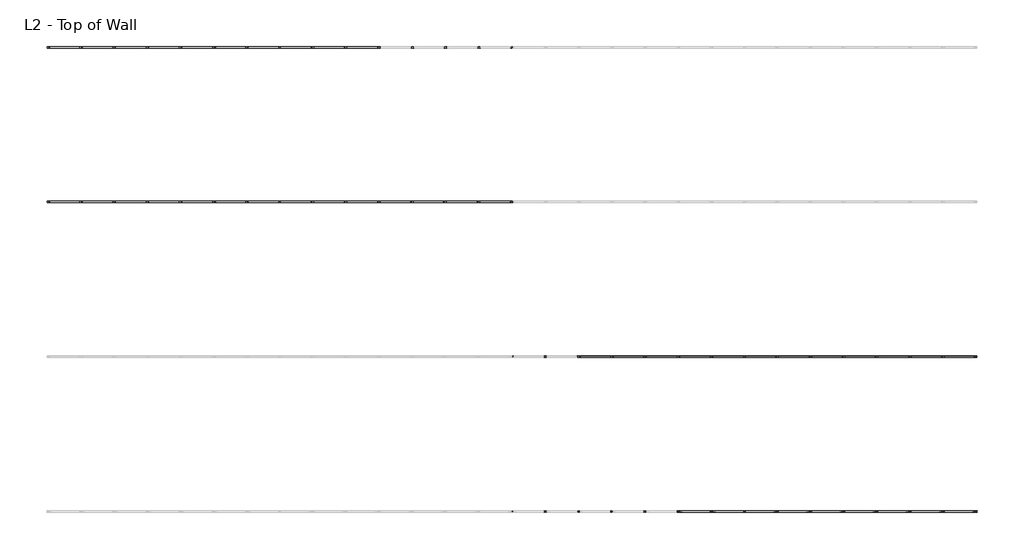
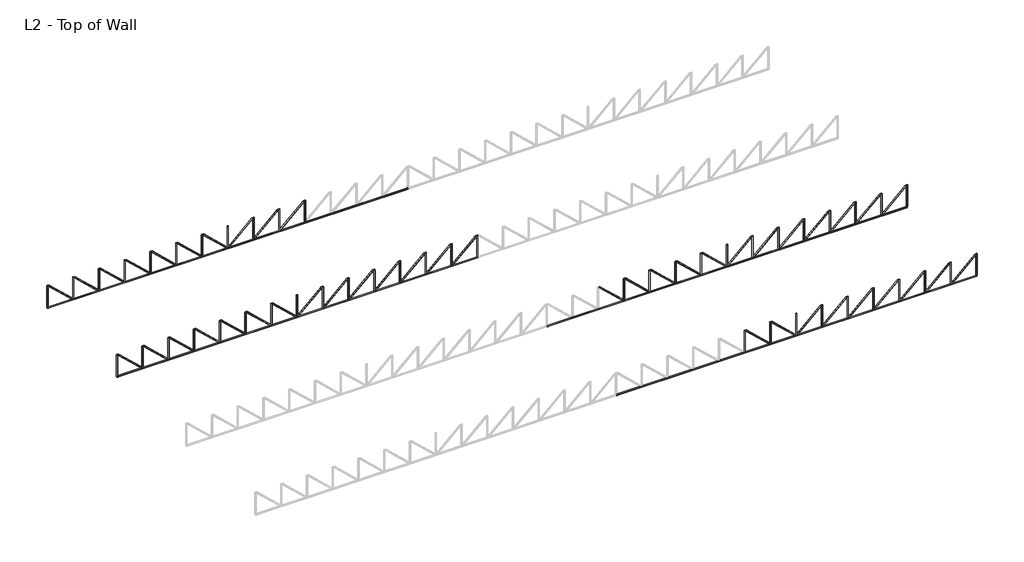
# One storey, part 3 of 4: 97 beams.
"""IFC4 building model written with IfcOpenShell, lengths in millimetres."""

import ifcopenshell
import ifcopenshell.guid

model = None  # the IFC model being written
_history = None  # IfcOwnerHistory: only IFC2X3 demands one
_inside = {}  # id of a spatial element -> (the spatial element, [elements in it])
_under = {}  # id of a project, library or spatial element -> (it, [spatial elements below it])
_declared = {}  # id of a project -> (the project, [libraries it declares])
_typed = {}  # id of a type object -> (the type object, [elements of that type])
_made_of = {}  # id of a material, layer set ... -> (it, [elements and type objects made of it])


def new_model(schema):
    """Start an empty IFC model of exactly this schema.

    Asked for "IFC4X3", IfcOpenShell would pick the latest addendum, in which some entities
    have other attributes; the version numbers below select the first issue.
    IFC2X3 requires an IfcOwnerHistory on every rooted entity: one is made here for all.
    """
    global model, _history
    if schema == "IFC4X3":
        model = ifcopenshell.file(schema_version=(4, 3, 0, 0))
    else:
        model = ifcopenshell.file(schema=schema)
    _inside.clear()
    _under.clear()
    _declared.clear()
    _typed.clear()
    _made_of.clear()
    _history = None
    if model.schema == "IFC2X3":
        org = make("IfcOrganization", Name="unknown")
        user = make(
            "IfcPersonAndOrganization",
            ThePerson=make("IfcPerson", FamilyName="unknown"),
            TheOrganization=org,
        )
        app = make(
            "IfcApplication",
            ApplicationDeveloper=org,
            Version="unknown",
            ApplicationFullName="unknown",
            ApplicationIdentifier="unknown",
        )
        _history = make(
            "IfcOwnerHistory",
            OwningUser=user,
            OwningApplication=app,
            ChangeAction="ADDED",
            CreationDate=0,
        )
    return model


def make(cls, **values):
    """One entity of the class cls with the attributes given. An attribute that is None is left unset."""
    return model.create_entity(
        cls, **{name: value for name, value in values.items() if value is not None}
    )


def rooted(cls, **values):
    """An entity with a GlobalId (a new one), such as an element, a storey or a relation."""
    return make(cls, GlobalId=ifcopenshell.guid.new(), OwnerHistory=_history, **values)


def si_unit(unit_type, name, prefix=None):
    """IfcSIUnit, for example si_unit("LENGTHUNIT", "METRE", prefix="MILLI")."""
    return make("IfcSIUnit", UnitType=unit_type, Prefix=prefix, Name=name)


def assignment(units):
    """IfcUnitAssignment: the units of a project."""
    return None if units is None else make("IfcUnitAssignment", Units=units)


def point(xyz):
    """IfcCartesianPoint."""
    return None if xyz is None else make("IfcCartesianPoint", Coordinates=xyz)


def direction(xyz):
    """IfcDirection."""
    return None if xyz is None else make("IfcDirection", DirectionRatios=xyz)


def frame(location, z_axis=None, x_axis=None):
    """IfcAxis2Placement3D, a coordinate frame: its origin and axes. An axis left out is left unset."""
    return make(
        "IfcAxis2Placement3D",
        Location=point(location),
        Axis=direction(z_axis),
        RefDirection=direction(x_axis),
    )


def frame_2d(location, x_axis=None):
    """IfcAxis2Placement2D, a coordinate frame in the plane: its origin and x axis."""
    return make(
        "IfcAxis2Placement2D", Location=point(location), RefDirection=direction(x_axis)
    )


def origin():
    """The frame at (0, 0, 0) with its axes left unset."""
    return frame((0.0, 0.0, 0.0))


def origin_2d():
    """The frame at (0, 0) in the plane with its x axis left unset."""
    return frame_2d((0.0, 0.0))


def place(relative_to, where):
    """IfcLocalPlacement: puts the frame where relative to a parent placement (None: the world)."""
    return make(
        "IfcLocalPlacement", PlacementRelTo=relative_to, RelativePlacement=where
    )


def context(
    kind, dimensions, precision=None, world=None, true_north=None, identifier=None
):
    """IfcGeometricRepresentationContext, for example the 3D "Model" context."""
    return make(
        "IfcGeometricRepresentationContext",
        ContextIdentifier=identifier,
        ContextType=kind,
        CoordinateSpaceDimension=dimensions,
        Precision=precision,
        WorldCoordinateSystem=world,
        TrueNorth=true_north,
    )


def project(units=None, contexts=None):
    """IfcProject with its units and contexts."""
    return rooted(
        "IfcProject",
        Name="project",
        RepresentationContexts=contexts,
        UnitsInContext=assignment(units),
    )


def spatial(cls, under=None, at=None, **own):
    """A site, building, storey or space (cls), placed at a placement, below another one or the project."""
    s = rooted(cls, ObjectPlacement=at, **own)
    if under is not None:
        _under.setdefault(under.id(), (under, []))[1].append(s)
    return s


def circle_curve(where, radius):
    """IfcCircle in the frame where."""
    return make("IfcCircle", Position=where, Radius=radius)


def trimmed(basis, trim1, trim2, sense, master):
    """IfcTrimmedCurve: the piece of a basis curve between two trims."""
    return make(
        "IfcTrimmedCurve",
        BasisCurve=basis,
        Trim1=trim1,
        Trim2=trim2,
        SenseAgreement=sense,
        MasterRepresentation=master,
    )


def segment(curve, same_sense, transition):
    """IfcCompositeCurveSegment."""
    return make(
        "IfcCompositeCurveSegment",
        Transition=transition,
        SameSense=same_sense,
        ParentCurve=curve,
    )


def composite_curve(segments, self_intersect=None):
    """IfcCompositeCurve: segments joined end to end."""
    return make("IfcCompositeCurve", Segments=segments, SelfIntersect=self_intersect)


def outline(outer, holes=None, kind="AREA"):
    """IfcArbitraryClosedProfileDef: a profile drawn as a closed curve; with holes, ...WithVoids."""
    if holes is None:
        return make("IfcArbitraryClosedProfileDef", ProfileType=kind, OuterCurve=outer)
    return make(
        "IfcArbitraryProfileDefWithVoids",
        ProfileType=kind,
        OuterCurve=outer,
        InnerCurves=holes,
    )


def extrude(swept, where, along, depth):
    """IfcExtrudedAreaSolid: the profile swept, set in the frame where, extruded along a direction by depth."""
    return make(
        "IfcExtrudedAreaSolid",
        SweptArea=swept,
        Position=where,
        ExtrudedDirection=direction(along),
        Depth=depth,
    )


def shape(context_of_items, identifier, shape_type, items):
    """IfcShapeRepresentation: the items that make up one representation, for example the "Body"."""
    return make(
        "IfcShapeRepresentation",
        ContextOfItems=context_of_items,
        RepresentationIdentifier=identifier,
        RepresentationType=shape_type,
        Items=items,
    )


def source(mapping_origin, context_of_items, identifier, shape_type, items):
    """IfcRepresentationMap: a shape defined once, which mapped items show again and again."""
    return make(
        "IfcRepresentationMap",
        MappingOrigin=mapping_origin,
        MappedRepresentation=shape(context_of_items, identifier, shape_type, items),
    )


def transform(
    local_origin,
    x_axis=None,
    y_axis=None,
    z_axis=None,
    scale=None,
    scale2=None,
    scale3=None,
    uniform=True,
):
    """IfcCartesianTransformationOperator3D, or its non-uniform kind. x_axis, y_axis, z_axis: its Axis1, 2, 3."""
    if uniform:
        return make(
            "IfcCartesianTransformationOperator3D",
            Axis1=direction(x_axis),
            Axis2=direction(y_axis),
            LocalOrigin=point(local_origin),
            Scale=scale,
            Axis3=direction(z_axis),
        )
    return make(
        "IfcCartesianTransformationOperator3DnonUniform",
        Axis1=direction(x_axis),
        Axis2=direction(y_axis),
        LocalOrigin=point(local_origin),
        Scale=scale,
        Axis3=direction(z_axis),
        Scale2=scale2,
        Scale3=scale3,
    )


def mapped(mapping_source, mapping_target):
    """IfcMappedItem: shows the shape of a source again, moved by a transform."""
    return make(
        "IfcMappedItem", MappingSource=mapping_source, MappingTarget=mapping_target
    )


def made_of(thing, what):
    """Note that an element or type object is made of a material, layer set ...; save() writes the relation."""
    if what is not None:
        _made_of.setdefault(what.id(), (what, []))[1].append(thing)
    return thing


def element(
    cls,
    number,
    at=None,
    inside=None,
    cuts=None,
    type_object=None,
    material=None,
    context=None,
    identifier="Body",
    shape_type=None,
    held_by="IfcProductDefinitionShape",
    body=None,
    shapes=None,
    **own,
):
    """One element of the class cls, such as IfcWall. Its Tag is "e" and its number.

    at: its placement. inside: the storey or other place that contains it. cuts: it is an
    opening in that element (IfcRelVoidsElement). A single representation is given by context,
    identifier, shape_type and body (its items); several are given by shapes. held_by: the class
    of the entity that holds the representations. save() writes the other relations.
    """
    e = rooted(cls, Tag="e%d" % number, ObjectPlacement=at, **own)
    if body is not None:
        shapes = [shape(context, identifier, shape_type, body)]
    if shapes is not None:
        e.Representation = make(held_by, Representations=shapes)
    if inside is not None:
        _inside.setdefault(inside.id(), (inside, []))[1].append(e)
    if cuts is not None:
        rooted(
            "IfcRelVoidsElement", RelatingBuildingElement=cuts, RelatedOpeningElement=e
        )
    if type_object is not None:
        _typed.setdefault(type_object.id(), (type_object, []))[1].append(e)
    return made_of(e, material)


def aggregate(whole, parts):
    """IfcRelAggregates: a whole, such as a stair, and the parts it consists of."""
    return rooted("IfcRelAggregates", RelatingObject=whole, RelatedObjects=parts)


def save(model, path):
    """Write the relations noted so far, then the file.

    IfcRelAggregates (storeys below a building ...), IfcRelContainedInSpatialStructure (elements
    in a storey), IfcRelDefinesByType, IfcRelAssociatesMaterial and IfcRelDeclares: one each for
    every whole, place, type object, material and project.
    """
    for whole, parts in _under.values():
        aggregate(whole, parts)
    for where, things in _inside.values():
        rooted(
            "IfcRelContainedInSpatialStructure",
            RelatedElements=things,
            RelatingStructure=where,
        )
    for kind, things in _typed.values():
        rooted("IfcRelDefinesByType", RelatedObjects=things, RelatingType=kind)
    for what, things in _made_of.values():
        rooted("IfcRelAssociatesMaterial", RelatedObjects=things, RelatingMaterial=what)
    for by, libraries in _declared.values():
        rooted("IfcRelDeclares", RelatingContext=by, RelatedDefinitions=libraries)
    model.write(path)


def circular_hollow_sections_chs60_3x5_c94bd862(model_context):
    return source(origin(), model_context, "Body", "SweptSolid", [
        extrude(outline(composite_curve([segment(trimmed(circle_curve(origin_2d(), 30.15), [point((-30.15, 0.0))], [point((30.15, 0.0))], False, "CARTESIAN"), True, "CONTINUOUS"), segment(trimmed(circle_curve(origin_2d(), 30.15), [point((30.15, 0.0))], [point((-30.15, 0.0))], False, "CARTESIAN"), True, "CONTINUOUS")], self_intersect=False), holes=[composite_curve([segment(trimmed(circle_curve(origin_2d(), 25.15), [point((25.15, 0.0))], [point((-25.15, 0.0))], True, "CARTESIAN"), True, "CONTINUOUS"), segment(trimmed(circle_curve(origin_2d(), 25.15), [point((-25.15, 0.0))], [point((25.15, 0.0))], True, "CARTESIAN"), True, "CONTINUOUS")], self_intersect=False)]), frame((-557.0, 0.0, 0.0), z_axis=(1.0, 0.0, 0.0), x_axis=(0.0, 1.0, 0.0)), (0.0, 0.0, 1.0), 1114.0),
    ])


def circular_hollow_sections_chs60_3x5_b8a643cb(model_context):
    return source(origin(), model_context, "Body", "SweptSolid", [
        extrude(outline(composite_curve([segment(trimmed(circle_curve(origin_2d(), 30.15), [point((-30.15, 0.0))], [point((30.15, 0.0))], False, "CARTESIAN"), True, "CONTINUOUS"), segment(trimmed(circle_curve(origin_2d(), 30.15), [point((30.15, 0.0))], [point((-30.15, 0.0))], False, "CARTESIAN"), True, "CONTINUOUS")], self_intersect=False), holes=[composite_curve([segment(trimmed(circle_curve(origin_2d(), 25.15), [point((25.15, 0.0))], [point((-25.15, 0.0))], True, "CARTESIAN"), True, "CONTINUOUS"), segment(trimmed(circle_curve(origin_2d(), 25.15), [point((-25.15, 0.0))], [point((25.15, 0.0))], True, "CARTESIAN"), True, "CONTINUOUS")], self_intersect=False)]), frame((-790.0, 0.0, 0.0), z_axis=(1.0, 0.0, 0.0), x_axis=(0.0, 1.0, 0.0)), (0.0, 0.0, 1.0), 1580.0),
    ])


def circular_hollow_sections_chs60_3x5_ee2473de(model_context):
    return source(origin(), model_context, "Body", "SweptSolid", [
        extrude(outline(composite_curve([segment(trimmed(circle_curve(origin_2d(), 30.15), [point((-30.15, 0.0))], [point((30.15, 0.0))], False, "CARTESIAN"), True, "CONTINUOUS"), segment(trimmed(circle_curve(origin_2d(), 30.15), [point((30.15, 0.0))], [point((-30.15, 0.0))], False, "CARTESIAN"), True, "CONTINUOUS")], self_intersect=False), holes=[composite_curve([segment(trimmed(circle_curve(origin_2d(), 25.15), [point((25.15, 0.0))], [point((-25.15, 0.0))], True, "CARTESIAN"), True, "CONTINUOUS"), segment(trimmed(circle_curve(origin_2d(), 25.15), [point((-25.15, 0.0))], [point((25.15, 0.0))], True, "CARTESIAN"), True, "CONTINUOUS")], self_intersect=False)]), frame((-9000.0, 0.0, 0.0), z_axis=(1.0, 0.0, 0.0), x_axis=(0.0, 1.0, 0.0)), (0.0, 0.0, 1.0), 18000.0),
    ])


def circular_hollow_sections_chs60_3x5_7809bf4e(model_context):
    return source(origin(), model_context, "Body", "SweptSolid", [
        extrude(outline(composite_curve([segment(trimmed(circle_curve(origin_2d(), 30.15), [point((-30.15, 0.0))], [point((30.15, 0.0))], False, "CARTESIAN"), True, "CONTINUOUS"), segment(trimmed(circle_curve(origin_2d(), 30.15), [point((30.15, 0.0))], [point((-30.15, 0.0))], False, "CARTESIAN"), True, "CONTINUOUS")], self_intersect=False), holes=[composite_curve([segment(trimmed(circle_curve(origin_2d(), 25.15), [point((25.15, 0.0))], [point((-25.15, 0.0))], True, "CARTESIAN"), True, "CONTINUOUS"), segment(trimmed(circle_curve(origin_2d(), 25.15), [point((-25.15, 0.0))], [point((25.15, 0.0))], True, "CARTESIAN"), True, "CONTINUOUS")], self_intersect=False)]), frame((-600.0, 0.0, 0.0), z_axis=(1.0, 0.0, 0.0), x_axis=(0.0, 1.0, 0.0)), (0.0, 0.0, 1.0), 1157.0),
    ])


model = new_model("IFC4")

# Units and contexts
model_context = context("Model", 3, world=origin())
ifc_project = project(units=[si_unit("LENGTHUNIT", "METRE", prefix="MILLI")], contexts=[model_context])

# Site, building, storey
site = spatial("IfcSite", under=ifc_project)
building = spatial("IfcBuilding", under=site)
storey = spatial("IfcBuildingStorey", under=building, Name="L2 - Top of Wall", Elevation=6600.0)

# Beams
placement = place(None, origin())
circular_hollow_sections_chs60_3x5_shape = circular_hollow_sections_chs60_3x5_c94bd862(model_context)
element("IfcBeam", 1, ObjectType="Circular Hollow Sections : CHS60.3x5", at=placement, inside=storey, context=model_context, shape_type="MappedRepresentation", body=[
    mapped(circular_hollow_sections_chs60_3x5_shape, transform((27576.1803686, 941.2380918, 7200.0), x_axis=(0.0, 0.0, 1.0), y_axis=(0.0, -1.0, 0.0), z_axis=(1.0, 0.0, 0.0))),
])
element("IfcBeam", 2, ObjectType="Circular Hollow Sections : CHS60.3x5", at=placement, inside=storey, context=model_context, shape_type="MappedRepresentation", body=[
    mapped(circular_hollow_sections_chs60_3x5_shape, transform((12147.60894, 941.2380918, 7200.0), x_axis=(0.0, 0.0, 1.0), y_axis=(0.0, -1.0, 0.0), z_axis=(1.0, 0.0, 0.0))),
])
element("IfcBeam", 3, ObjectType="Circular Hollow Sections : CHS60.3x5", at=placement, inside=storey, context=model_context, shape_type="MappedRepresentation", body=[
    mapped(circular_hollow_sections_chs60_3x5_shape, transform((26290.4660829, 941.2380918, 7200.0), x_axis=(0.0, 0.0, 1.0), y_axis=(0.0, -1.0, 0.0), z_axis=(1.0, 0.0, 0.0))),
])
element("IfcBeam", 4, ObjectType="Circular Hollow Sections : CHS60.3x5", at=placement, inside=storey, context=model_context, shape_type="MappedRepresentation", body=[
    mapped(circular_hollow_sections_chs60_3x5_shape, transform((13433.3232257, 941.2380918, 7200.0), x_axis=(0.0, 0.0, 1.0), y_axis=(0.0, -1.0, 0.0), z_axis=(1.0, 0.0, 0.0))),
])
element("IfcBeam", 5, ObjectType="Circular Hollow Sections : CHS60.3x5", at=placement, inside=storey, context=model_context, shape_type="MappedRepresentation", body=[
    mapped(circular_hollow_sections_chs60_3x5_shape, transform((25004.7517972, 941.2380918, 7200.0), x_axis=(0.0, 0.0, 1.0), y_axis=(0.0, -1.0, 0.0), z_axis=(1.0, 0.0, 0.0))),
])
element("IfcBeam", 6, ObjectType="Circular Hollow Sections : CHS60.3x5", at=placement, inside=storey, context=model_context, shape_type="MappedRepresentation", body=[
    mapped(circular_hollow_sections_chs60_3x5_shape, transform((14719.0375115, 941.2380918, 7200.0), x_axis=(0.0, 0.0, 1.0), y_axis=(0.0, -1.0, 0.0), z_axis=(1.0, 0.0, 0.0))),
])
element("IfcBeam", 7, ObjectType="Circular Hollow Sections : CHS60.3x5", at=placement, inside=storey, context=model_context, shape_type="MappedRepresentation", body=[
    mapped(circular_hollow_sections_chs60_3x5_shape, transform((23719.0375115, 941.2380918, 7200.0), x_axis=(0.0, 0.0, 1.0), y_axis=(0.0, -1.0, 0.0), z_axis=(1.0, 0.0, 0.0))),
])
element("IfcBeam", 8, ObjectType="Circular Hollow Sections : CHS60.3x5", at=placement, inside=storey, context=model_context, shape_type="MappedRepresentation", body=[
    mapped(circular_hollow_sections_chs60_3x5_shape, transform((22433.3232257, 941.2380918, 7200.0), x_axis=(0.0, 0.0, 1.0), y_axis=(0.0, -1.0, 0.0), z_axis=(1.0, 0.0, 0.0))),
])
element("IfcBeam", 9, ObjectType="Circular Hollow Sections : CHS60.3x5", at=placement, inside=storey, context=model_context, shape_type="MappedRepresentation", body=[
    mapped(circular_hollow_sections_chs60_3x5_shape, transform((28861.8946543, 941.2380918, 7200.0), x_axis=(0.0, 0.0, 1.0), y_axis=(0.0, -1.0, 0.0), z_axis=(1.0, 0.0, 0.0))),
])
element("IfcBeam", 10, ObjectType="Circular Hollow Sections : CHS60.3x5", at=placement, inside=storey, context=model_context, shape_type="MappedRepresentation", body=[
    mapped(circular_hollow_sections_chs60_3x5_shape, transform((21147.60894, 941.2380918, 7200.0), x_axis=(0.0, 0.0, 1.0), y_axis=(0.0, -1.0, 0.0), z_axis=(1.0, 0.0, 0.0))),
])
element("IfcBeam", 11, ObjectType="Circular Hollow Sections : CHS60.3x5", at=placement, inside=storey, context=model_context, shape_type="MappedRepresentation", body=[
    mapped(circular_hollow_sections_chs60_3x5_shape, transform((16004.7517972, 941.2380918, 7200.0), x_axis=(0.0, 0.0, 1.0), y_axis=(0.0, -1.0, 0.0), z_axis=(1.0, 0.0, 0.0))),
])
element("IfcBeam", 12, ObjectType="Circular Hollow Sections : CHS60.3x5", at=placement, inside=storey, context=model_context, shape_type="MappedRepresentation", body=[
    mapped(circular_hollow_sections_chs60_3x5_shape, transform((17290.4660829, 941.2380918, 7200.0), x_axis=(0.0, 0.0, 1.0), y_axis=(0.0, -1.0, 0.0), z_axis=(1.0, 0.0, 0.0))),
])
element("IfcBeam", 13, ObjectType="Circular Hollow Sections : CHS60.3x5", at=placement, inside=storey, context=model_context, shape_type="MappedRepresentation", body=[
    mapped(circular_hollow_sections_chs60_3x5_shape, transform((10861.8946543, 941.2380918, 7200.0), x_axis=(0.0, 0.0, 1.0), y_axis=(0.0, -1.0, 0.0), z_axis=(1.0, 0.0, 0.0))),
])
element("IfcBeam", 14, ObjectType="Circular Hollow Sections : CHS60.3x5", at=placement, inside=storey, context=model_context, shape_type="MappedRepresentation", body=[
    mapped(circular_hollow_sections_chs60_3x5_shape, transform((18576.1803686, 941.2380918, 7200.0), x_axis=(0.0, 0.0, 1.0), y_axis=(0.0, -1.0, 0.0), z_axis=(1.0, 0.0, 0.0))),
])
element("IfcBeam", 15, ObjectType="Circular Hollow Sections : CHS60.3x5", at=placement, inside=storey, context=model_context, shape_type="MappedRepresentation", body=[
    mapped(circular_hollow_sections_chs60_3x5_shape, transform((19861.8946543, 941.2380918, 7200.0), x_axis=(0.0, 0.0, 1.0), y_axis=(0.0, -1.0, 0.0), z_axis=(1.0, 0.0, 0.0))),
])
element("IfcBeam", 16, ObjectType="Circular Hollow Sections : CHS60.3x5", at=placement, inside=storey, context=model_context, shape_type="MappedRepresentation", body=[
    mapped(circular_hollow_sections_chs60_3x5_shape, transform((12147.60894, 6941.2380918, 7200.0), x_axis=(0.0, 0.0, 1.0), y_axis=(0.0, -1.0, 0.0), z_axis=(1.0, 0.0, 0.0))),
])
element("IfcBeam", 17, ObjectType="Circular Hollow Sections : CHS60.3x5", at=placement, inside=storey, context=model_context, shape_type="MappedRepresentation", body=[
    mapped(circular_hollow_sections_chs60_3x5_shape, transform((13433.3232257, 6941.2380918, 7200.0), x_axis=(0.0, 0.0, 1.0), y_axis=(0.0, -1.0, 0.0), z_axis=(1.0, 0.0, 0.0))),
])
element("IfcBeam", 18, ObjectType="Circular Hollow Sections : CHS60.3x5", at=placement, inside=storey, context=model_context, shape_type="MappedRepresentation", body=[
    mapped(circular_hollow_sections_chs60_3x5_shape, transform((14719.0375115, 6941.2380918, 7200.0), x_axis=(0.0, 0.0, 1.0), y_axis=(0.0, -1.0, 0.0), z_axis=(1.0, 0.0, 0.0))),
])
element("IfcBeam", 19, ObjectType="Circular Hollow Sections : CHS60.3x5", at=placement, inside=storey, context=model_context, shape_type="MappedRepresentation", body=[
    mapped(circular_hollow_sections_chs60_3x5_shape, transform((23719.0375115, 6941.2380918, 7200.0), x_axis=(0.0, 0.0, 1.0), y_axis=(0.0, -1.0, 0.0), z_axis=(1.0, 0.0, 0.0))),
])
element("IfcBeam", 20, ObjectType="Circular Hollow Sections : CHS60.3x5", at=placement, inside=storey, context=model_context, shape_type="MappedRepresentation", body=[
    mapped(circular_hollow_sections_chs60_3x5_shape, transform((22433.3232257, 6941.2380918, 7200.0), x_axis=(0.0, 0.0, 1.0), y_axis=(0.0, -1.0, 0.0), z_axis=(1.0, 0.0, 0.0))),
])
element("IfcBeam", 21, ObjectType="Circular Hollow Sections : CHS60.3x5", at=placement, inside=storey, context=model_context, shape_type="MappedRepresentation", body=[
    mapped(circular_hollow_sections_chs60_3x5_shape, transform((21147.60894, 6941.2380918, 7200.0), x_axis=(0.0, 0.0, 1.0), y_axis=(0.0, -1.0, 0.0), z_axis=(1.0, 0.0, 0.0))),
])
element("IfcBeam", 22, ObjectType="Circular Hollow Sections : CHS60.3x5", at=placement, inside=storey, context=model_context, shape_type="MappedRepresentation", body=[
    mapped(circular_hollow_sections_chs60_3x5_shape, transform((16004.7517972, 6941.2380918, 7200.0), x_axis=(0.0, 0.0, 1.0), y_axis=(0.0, -1.0, 0.0), z_axis=(1.0, 0.0, 0.0))),
])
element("IfcBeam", 23, ObjectType="Circular Hollow Sections : CHS60.3x5", at=placement, inside=storey, context=model_context, shape_type="MappedRepresentation", body=[
    mapped(circular_hollow_sections_chs60_3x5_shape, transform((17290.4660829, 6941.2380918, 7200.0), x_axis=(0.0, 0.0, 1.0), y_axis=(0.0, -1.0, 0.0), z_axis=(1.0, 0.0, 0.0))),
])
element("IfcBeam", 24, ObjectType="Circular Hollow Sections : CHS60.3x5", at=placement, inside=storey, context=model_context, shape_type="MappedRepresentation", body=[
    mapped(circular_hollow_sections_chs60_3x5_shape, transform((18576.1803686, 6941.2380918, 7200.0), x_axis=(0.0, 0.0, 1.0), y_axis=(0.0, -1.0, 0.0), z_axis=(1.0, 0.0, 0.0))),
])
element("IfcBeam", 25, ObjectType="Circular Hollow Sections : CHS60.3x5", at=placement, inside=storey, context=model_context, shape_type="MappedRepresentation", body=[
    mapped(circular_hollow_sections_chs60_3x5_shape, transform((19861.8946543, 6941.2380918, 7200.0), x_axis=(0.0, 0.0, 1.0), y_axis=(0.0, -1.0, 0.0), z_axis=(1.0, 0.0, 0.0))),
])
element("IfcBeam", 26, ObjectType="Circular Hollow Sections : CHS60.3x5", at=placement, inside=storey, context=model_context, shape_type="MappedRepresentation", body=[
    mapped(circular_hollow_sections_chs60_3x5_shape, transform((45576.1803686, -5058.7619082, 7200.0), x_axis=(0.0, 0.0, 1.0000000000000002), y_axis=(0.0, -1.0000000000000002, 0.0), z_axis=(1.0000000000000002, 0.0, 0.0))),
])
element("IfcBeam", 27, ObjectType="Circular Hollow Sections : CHS60.3x5", at=placement, inside=storey, context=model_context, shape_type="MappedRepresentation", body=[
    mapped(circular_hollow_sections_chs60_3x5_shape, transform((44290.4660829, -5058.7619082, 7200.0), x_axis=(0.0, 0.0, 1.0000000000000002), y_axis=(0.0, -1.0000000000000002, 0.0), z_axis=(1.0000000000000002, 0.0, 0.0))),
])
element("IfcBeam", 28, ObjectType="Circular Hollow Sections : CHS60.3x5", at=placement, inside=storey, context=model_context, shape_type="MappedRepresentation", body=[
    mapped(circular_hollow_sections_chs60_3x5_shape, transform((43004.7517972, -5058.7619082, 7200.0), x_axis=(0.0, 0.0, 1.0000000000000002), y_axis=(0.0, -1.0000000000000002, 0.0), z_axis=(1.0000000000000002, 0.0, 0.0))),
])
element("IfcBeam", 29, ObjectType="Circular Hollow Sections : CHS60.3x5", at=placement, inside=storey, context=model_context, shape_type="MappedRepresentation", body=[
    mapped(circular_hollow_sections_chs60_3x5_shape, transform((32719.0375115, -5058.7619082, 7200.0), x_axis=(0.0, 0.0, 1.0000000000000002), y_axis=(0.0, -1.0000000000000002, 0.0), z_axis=(1.0000000000000002, 0.0, 0.0))),
])
element("IfcBeam", 30, ObjectType="Circular Hollow Sections : CHS60.3x5", at=placement, inside=storey, context=model_context, shape_type="MappedRepresentation", body=[
    mapped(circular_hollow_sections_chs60_3x5_shape, transform((41719.0375115, -5058.7619082, 7200.0), x_axis=(0.0, 0.0, 1.0000000000000002), y_axis=(0.0, -1.0000000000000002, 0.0), z_axis=(1.0000000000000002, 0.0, 0.0))),
])
element("IfcBeam", 31, ObjectType="Circular Hollow Sections : CHS60.3x5", at=placement, inside=storey, context=model_context, shape_type="MappedRepresentation", body=[
    mapped(circular_hollow_sections_chs60_3x5_shape, transform((40433.3232257, -5058.7619082, 7200.0), x_axis=(0.0, 0.0, 1.0000000000000002), y_axis=(0.0, -1.0000000000000002, 0.0), z_axis=(1.0000000000000002, 0.0, 0.0))),
])
element("IfcBeam", 32, ObjectType="Circular Hollow Sections : CHS60.3x5", at=placement, inside=storey, context=model_context, shape_type="MappedRepresentation", body=[
    mapped(circular_hollow_sections_chs60_3x5_shape, transform((46861.8946543, -5058.7619082, 7200.0), x_axis=(0.0, 0.0, 1.0000000000000002), y_axis=(0.0, -1.0000000000000002, 0.0), z_axis=(1.0000000000000002, 0.0, 0.0))),
])
element("IfcBeam", 33, ObjectType="Circular Hollow Sections : CHS60.3x5", at=placement, inside=storey, context=model_context, shape_type="MappedRepresentation", body=[
    mapped(circular_hollow_sections_chs60_3x5_shape, transform((39147.60894, -5058.7619082, 7200.0), x_axis=(0.0, 0.0, 1.0000000000000002), y_axis=(0.0, -1.0000000000000002, 0.0), z_axis=(1.0000000000000002, 0.0, 0.0))),
])
element("IfcBeam", 34, ObjectType="Circular Hollow Sections : CHS60.3x5", at=placement, inside=storey, context=model_context, shape_type="MappedRepresentation", body=[
    mapped(circular_hollow_sections_chs60_3x5_shape, transform((34004.7517972, -5058.7619082, 7200.0), x_axis=(0.0, 0.0, 1.0000000000000002), y_axis=(0.0, -1.0000000000000002, 0.0), z_axis=(1.0000000000000002, 0.0, 0.0))),
])
element("IfcBeam", 35, ObjectType="Circular Hollow Sections : CHS60.3x5", at=placement, inside=storey, context=model_context, shape_type="MappedRepresentation", body=[
    mapped(circular_hollow_sections_chs60_3x5_shape, transform((35290.4660829, -5058.7619082, 7200.0), x_axis=(0.0, 0.0, 1.0000000000000002), y_axis=(0.0, -1.0000000000000002, 0.0), z_axis=(1.0000000000000002, 0.0, 0.0))),
])
element("IfcBeam", 36, ObjectType="Circular Hollow Sections : CHS60.3x5", at=placement, inside=storey, context=model_context, shape_type="MappedRepresentation", body=[
    mapped(circular_hollow_sections_chs60_3x5_shape, transform((36576.1803686, -5058.7619082, 7200.0), x_axis=(0.0, 0.0, 1.0000000000000002), y_axis=(0.0, -1.0000000000000002, 0.0), z_axis=(1.0000000000000002, 0.0, 0.0))),
])
element("IfcBeam", 37, ObjectType="Circular Hollow Sections : CHS60.3x5", at=placement, inside=storey, context=model_context, shape_type="MappedRepresentation", body=[
    mapped(circular_hollow_sections_chs60_3x5_shape, transform((37861.8946543, -5058.7619082, 7200.0), x_axis=(0.0, 0.0, 1.0000000000000002), y_axis=(0.0, -1.0000000000000002, 0.0), z_axis=(1.0000000000000002, 0.0, 0.0))),
])
element("IfcBeam", 38, ObjectType="Circular Hollow Sections : CHS60.3x5", at=placement, inside=storey, context=model_context, shape_type="MappedRepresentation", body=[
    mapped(circular_hollow_sections_chs60_3x5_shape, transform((45576.1803686, -11058.7619082, 7200.0), x_axis=(0.0, 0.0, 1.0000000000000002), y_axis=(0.0, -1.0000000000000002, 0.0), z_axis=(1.0000000000000002, 0.0, 0.0))),
])
element("IfcBeam", 39, ObjectType="Circular Hollow Sections : CHS60.3x5", at=placement, inside=storey, context=model_context, shape_type="MappedRepresentation", body=[
    mapped(circular_hollow_sections_chs60_3x5_shape, transform((44290.4660829, -11058.7619082, 7200.0), x_axis=(0.0, 0.0, 1.0000000000000002), y_axis=(0.0, -1.0000000000000002, 0.0), z_axis=(1.0000000000000002, 0.0, 0.0))),
])
element("IfcBeam", 40, ObjectType="Circular Hollow Sections : CHS60.3x5", at=placement, inside=storey, context=model_context, shape_type="MappedRepresentation", body=[
    mapped(circular_hollow_sections_chs60_3x5_shape, transform((43004.7517972, -11058.7619082, 7200.0), x_axis=(0.0, 0.0, 1.0000000000000002), y_axis=(0.0, -1.0000000000000002, 0.0), z_axis=(1.0000000000000002, 0.0, 0.0))),
])
element("IfcBeam", 41, ObjectType="Circular Hollow Sections : CHS60.3x5", at=placement, inside=storey, context=model_context, shape_type="MappedRepresentation", body=[
    mapped(circular_hollow_sections_chs60_3x5_shape, transform((41719.0375115, -11058.7619082, 7200.0), x_axis=(0.0, 0.0, 1.0000000000000002), y_axis=(0.0, -1.0000000000000002, 0.0), z_axis=(1.0000000000000002, 0.0, 0.0))),
])
element("IfcBeam", 42, ObjectType="Circular Hollow Sections : CHS60.3x5", at=placement, inside=storey, context=model_context, shape_type="MappedRepresentation", body=[
    mapped(circular_hollow_sections_chs60_3x5_shape, transform((40433.3232257, -11058.7619082, 7200.0), x_axis=(0.0, 0.0, 1.0000000000000002), y_axis=(0.0, -1.0000000000000002, 0.0), z_axis=(1.0000000000000002, 0.0, 0.0))),
])
element("IfcBeam", 43, ObjectType="Circular Hollow Sections : CHS60.3x5", at=placement, inside=storey, context=model_context, shape_type="MappedRepresentation", body=[
    mapped(circular_hollow_sections_chs60_3x5_shape, transform((46861.8946543, -11058.7619082, 7200.0), x_axis=(0.0, 0.0, 1.0000000000000002), y_axis=(0.0, -1.0000000000000002, 0.0), z_axis=(1.0000000000000002, 0.0, 0.0))),
])
element("IfcBeam", 44, ObjectType="Circular Hollow Sections : CHS60.3x5", at=placement, inside=storey, context=model_context, shape_type="MappedRepresentation", body=[
    mapped(circular_hollow_sections_chs60_3x5_shape, transform((39147.60894, -11058.7619082, 7200.0), x_axis=(0.0, 0.0, 1.0000000000000002), y_axis=(0.0, -1.0000000000000002, 0.0), z_axis=(1.0000000000000002, 0.0, 0.0))),
])
element("IfcBeam", 45, ObjectType="Circular Hollow Sections : CHS60.3x5", at=placement, inside=storey, context=model_context, shape_type="MappedRepresentation", body=[
    mapped(circular_hollow_sections_chs60_3x5_shape, transform((35290.4660829, -11058.7619082, 7200.0), x_axis=(0.0, 0.0, 1.0000000000000002), y_axis=(0.0, -1.0000000000000002, 0.0), z_axis=(1.0000000000000002, 0.0, 0.0))),
])
element("IfcBeam", 46, ObjectType="Circular Hollow Sections : CHS60.3x5", at=placement, inside=storey, context=model_context, shape_type="MappedRepresentation", body=[
    mapped(circular_hollow_sections_chs60_3x5_shape, transform((36576.1803686, -11058.7619082, 7200.0), x_axis=(0.0, 0.0, 1.0000000000000002), y_axis=(0.0, -1.0000000000000002, 0.0), z_axis=(1.0000000000000002, 0.0, 0.0))),
])
element("IfcBeam", 47, ObjectType="Circular Hollow Sections : CHS60.3x5", at=placement, inside=storey, context=model_context, shape_type="MappedRepresentation", body=[
    mapped(circular_hollow_sections_chs60_3x5_shape, transform((37861.8946543, -11058.7619082, 7200.0), x_axis=(0.0, 0.0, 1.0000000000000002), y_axis=(0.0, -1.0000000000000002, 0.0), z_axis=(1.0000000000000002, 0.0, 0.0))),
])
circular_hollow_sections_chs60_3x5_2_shape = circular_hollow_sections_chs60_3x5_b8a643cb(model_context)
element("IfcBeam", 48, ObjectType="Circular Hollow Sections : CHS60.3x5", at=placement, inside=storey, context=model_context, shape_type="MappedRepresentation", body=[
    mapped(circular_hollow_sections_chs60_3x5_2_shape, transform((26933.3232257, 941.2380918, 7200.0), x_axis=(0.7310552682428697, 0.0, 0.6823182503600105), y_axis=(0.0, -1.0, 0.0), z_axis=(0.6823182503600105, 0.0, -0.7310552682428697))),
])
element("IfcBeam", 49, ObjectType="Circular Hollow Sections : CHS60.3x5", at=placement, inside=storey, context=model_context, shape_type="MappedRepresentation", body=[
    mapped(circular_hollow_sections_chs60_3x5_2_shape, transform((12790.4660829, 941.2380918, 7200.0), x_axis=(0.7310552682428691, 0.0, -0.6823182503600111), y_axis=(0.0, -1.0, 0.0), z_axis=(-0.6823182503600111, 0.0, -0.7310552682428691))),
])
element("IfcBeam", 50, ObjectType="Circular Hollow Sections : CHS60.3x5", at=placement, inside=storey, context=model_context, shape_type="MappedRepresentation", body=[
    mapped(circular_hollow_sections_chs60_3x5_2_shape, transform((25647.60894, 941.2380918, 7200.0), x_axis=(0.7310552682428697, 0.0, 0.6823182503600105), y_axis=(0.0, -1.0, 0.0), z_axis=(0.6823182503600105, 0.0, -0.7310552682428697))),
])
element("IfcBeam", 51, ObjectType="Circular Hollow Sections : CHS60.3x5", at=placement, inside=storey, context=model_context, shape_type="MappedRepresentation", body=[
    mapped(circular_hollow_sections_chs60_3x5_2_shape, transform((14076.1803686, 941.2380918, 7200.0), x_axis=(0.7310552682428691, 0.0, -0.6823182503600111), y_axis=(0.0, -1.0, 0.0), z_axis=(-0.6823182503600111, 0.0, -0.7310552682428691))),
])
element("IfcBeam", 52, ObjectType="Circular Hollow Sections : CHS60.3x5", at=placement, inside=storey, context=model_context, shape_type="MappedRepresentation", body=[
    mapped(circular_hollow_sections_chs60_3x5_2_shape, transform((24361.8946543, 941.2380918, 7200.0), x_axis=(0.7310552682428697, 0.0, 0.6823182503600105), y_axis=(0.0, -1.0, 0.0), z_axis=(0.6823182503600105, 0.0, -0.7310552682428697))),
])
element("IfcBeam", 53, ObjectType="Circular Hollow Sections : CHS60.3x5", at=placement, inside=storey, context=model_context, shape_type="MappedRepresentation", body=[
    mapped(circular_hollow_sections_chs60_3x5_2_shape, transform((15361.8946543, 941.2380918, 7200.0), x_axis=(0.7310552682428691, 0.0, -0.6823182503600111), y_axis=(0.0, -1.0, 0.0), z_axis=(-0.6823182503600111, 0.0, -0.7310552682428691))),
])
element("IfcBeam", 54, ObjectType="Circular Hollow Sections : CHS60.3x5", at=placement, inside=storey, context=model_context, shape_type="MappedRepresentation", body=[
    mapped(circular_hollow_sections_chs60_3x5_2_shape, transform((23076.1803686, 941.2380918, 7200.0), x_axis=(0.7310552682428697, 0.0, 0.6823182503600105), y_axis=(0.0, -1.0, 0.0), z_axis=(0.6823182503600105, 0.0, -0.7310552682428697))),
])
element("IfcBeam", 55, ObjectType="Circular Hollow Sections : CHS60.3x5", at=placement, inside=storey, context=model_context, shape_type="MappedRepresentation", body=[
    mapped(circular_hollow_sections_chs60_3x5_2_shape, transform((21790.4660829, 941.2380918, 7200.0), x_axis=(0.7310552682428697, 0.0, 0.6823182503600105), y_axis=(0.0, -1.0, 0.0), z_axis=(0.6823182503600105, 0.0, -0.7310552682428697))),
])
element("IfcBeam", 56, ObjectType="Circular Hollow Sections : CHS60.3x5", at=placement, inside=storey, context=model_context, shape_type="MappedRepresentation", body=[
    mapped(circular_hollow_sections_chs60_3x5_2_shape, transform((28219.0375115, 941.2380918, 7200.0), x_axis=(0.7310552682428697, 0.0, 0.6823182503600105), y_axis=(0.0, -1.0, 0.0), z_axis=(0.6823182503600105, 0.0, -0.7310552682428697))),
])
element("IfcBeam", 57, ObjectType="Circular Hollow Sections : CHS60.3x5", at=placement, inside=storey, context=model_context, shape_type="MappedRepresentation", body=[
    mapped(circular_hollow_sections_chs60_3x5_2_shape, transform((20504.7517972, 941.2380918, 7200.0), x_axis=(0.7310552682428697, 0.0, 0.6823182503600105), y_axis=(0.0, -1.0, 0.0), z_axis=(0.6823182503600105, 0.0, -0.7310552682428697))),
])
element("IfcBeam", 58, ObjectType="Circular Hollow Sections : CHS60.3x5", at=placement, inside=storey, context=model_context, shape_type="MappedRepresentation", body=[
    mapped(circular_hollow_sections_chs60_3x5_2_shape, transform((16647.60894, 941.2380918, 7200.0), x_axis=(0.7310552682428691, 0.0, -0.6823182503600111), y_axis=(0.0, -1.0, 0.0), z_axis=(-0.6823182503600111, 0.0, -0.7310552682428691))),
])
element("IfcBeam", 59, ObjectType="Circular Hollow Sections : CHS60.3x5", at=placement, inside=storey, context=model_context, shape_type="MappedRepresentation", body=[
    mapped(circular_hollow_sections_chs60_3x5_2_shape, transform((17933.3232257, 941.2380918, 7200.0), x_axis=(0.7310552682428691, 0.0, -0.6823182503600111), y_axis=(0.0, -1.0, 0.0), z_axis=(-0.6823182503600111, 0.0, -0.7310552682428691))),
])
element("IfcBeam", 60, ObjectType="Circular Hollow Sections : CHS60.3x5", at=placement, inside=storey, context=model_context, shape_type="MappedRepresentation", body=[
    mapped(circular_hollow_sections_chs60_3x5_2_shape, transform((11504.7517972, 941.2380918, 7200.0), x_axis=(0.7310552682428691, 0.0, -0.6823182503600111), y_axis=(0.0, -1.0, 0.0), z_axis=(-0.6823182503600111, 0.0, -0.7310552682428691))),
])
element("IfcBeam", 61, ObjectType="Circular Hollow Sections : CHS60.3x5", at=placement, inside=storey, context=model_context, shape_type="MappedRepresentation", body=[
    mapped(circular_hollow_sections_chs60_3x5_2_shape, transform((19219.0375115, 941.2380918, 7200.0), x_axis=(0.7310552682428686, 0.0, -0.6823182503600118), y_axis=(0.0, -1.0, 0.0), z_axis=(-0.6823182503600118, 0.0, -0.7310552682428686))),
])
element("IfcBeam", 62, ObjectType="Circular Hollow Sections : CHS60.3x5", at=placement, inside=storey, context=model_context, shape_type="MappedRepresentation", body=[
    mapped(circular_hollow_sections_chs60_3x5_2_shape, transform((12790.4660829, 6941.2380918, 7200.0), x_axis=(0.7310552682428691, 0.0, -0.6823182503600111), y_axis=(0.0, -1.0, 0.0), z_axis=(-0.6823182503600111, 0.0, -0.7310552682428691))),
])
element("IfcBeam", 63, ObjectType="Circular Hollow Sections : CHS60.3x5", at=placement, inside=storey, context=model_context, shape_type="MappedRepresentation", body=[
    mapped(circular_hollow_sections_chs60_3x5_2_shape, transform((14076.1803686, 6941.2380918, 7200.0), x_axis=(0.7310552682428691, 0.0, -0.6823182503600111), y_axis=(0.0, -1.0, 0.0), z_axis=(-0.6823182503600111, 0.0, -0.7310552682428691))),
])
element("IfcBeam", 64, ObjectType="Circular Hollow Sections : CHS60.3x5", at=placement, inside=storey, context=model_context, shape_type="MappedRepresentation", body=[
    mapped(circular_hollow_sections_chs60_3x5_2_shape, transform((15361.8946543, 6941.2380918, 7200.0), x_axis=(0.7310552682428691, 0.0, -0.6823182503600111), y_axis=(0.0, -1.0, 0.0), z_axis=(-0.6823182503600111, 0.0, -0.7310552682428691))),
])
element("IfcBeam", 65, ObjectType="Circular Hollow Sections : CHS60.3x5", at=placement, inside=storey, context=model_context, shape_type="MappedRepresentation", body=[
    mapped(circular_hollow_sections_chs60_3x5_2_shape, transform((23076.1803686, 6941.2380918, 7200.0), x_axis=(0.7310552682428697, 0.0, 0.6823182503600105), y_axis=(0.0, -1.0, 0.0), z_axis=(0.6823182503600105, 0.0, -0.7310552682428697))),
])
element("IfcBeam", 66, ObjectType="Circular Hollow Sections : CHS60.3x5", at=placement, inside=storey, context=model_context, shape_type="MappedRepresentation", body=[
    mapped(circular_hollow_sections_chs60_3x5_2_shape, transform((21790.4660829, 6941.2380918, 7200.0), x_axis=(0.7310552682428697, 0.0, 0.6823182503600105), y_axis=(0.0, -1.0, 0.0), z_axis=(0.6823182503600105, 0.0, -0.7310552682428697))),
])
element("IfcBeam", 67, ObjectType="Circular Hollow Sections : CHS60.3x5", at=placement, inside=storey, context=model_context, shape_type="MappedRepresentation", body=[
    mapped(circular_hollow_sections_chs60_3x5_2_shape, transform((20504.7517972, 6941.2380918, 7200.0), x_axis=(0.7310552682428697, 0.0, 0.6823182503600105), y_axis=(0.0, -1.0, 0.0), z_axis=(0.6823182503600105, 0.0, -0.7310552682428697))),
])
element("IfcBeam", 68, ObjectType="Circular Hollow Sections : CHS60.3x5", at=placement, inside=storey, context=model_context, shape_type="MappedRepresentation", body=[
    mapped(circular_hollow_sections_chs60_3x5_2_shape, transform((16647.60894, 6941.2380918, 7200.0), x_axis=(0.7310552682428691, 0.0, -0.6823182503600111), y_axis=(0.0, -1.0, 0.0), z_axis=(-0.6823182503600111, 0.0, -0.7310552682428691))),
])
element("IfcBeam", 69, ObjectType="Circular Hollow Sections : CHS60.3x5", at=placement, inside=storey, context=model_context, shape_type="MappedRepresentation", body=[
    mapped(circular_hollow_sections_chs60_3x5_2_shape, transform((17933.3232257, 6941.2380918, 7200.0), x_axis=(0.7310552682428691, 0.0, -0.6823182503600111), y_axis=(0.0, -1.0, 0.0), z_axis=(-0.6823182503600111, 0.0, -0.7310552682428691))),
])
element("IfcBeam", 70, ObjectType="Circular Hollow Sections : CHS60.3x5", at=placement, inside=storey, context=model_context, shape_type="MappedRepresentation", body=[
    mapped(circular_hollow_sections_chs60_3x5_2_shape, transform((11504.7517972, 6941.2380918, 7200.0), x_axis=(0.7310552682428691, 0.0, -0.6823182503600111), y_axis=(0.0, -1.0, 0.0), z_axis=(-0.6823182503600111, 0.0, -0.7310552682428691))),
])
element("IfcBeam", 71, ObjectType="Circular Hollow Sections : CHS60.3x5", at=placement, inside=storey, context=model_context, shape_type="MappedRepresentation", body=[
    mapped(circular_hollow_sections_chs60_3x5_2_shape, transform((19219.0375115, 6941.2380918, 7200.0), x_axis=(0.7310552682428686, 0.0, -0.6823182503600118), y_axis=(0.0, -1.0, 0.0), z_axis=(-0.6823182503600118, 0.0, -0.7310552682428686))),
])
element("IfcBeam", 72, ObjectType="Circular Hollow Sections : CHS60.3x5", at=placement, inside=storey, context=model_context, shape_type="MappedRepresentation", body=[
    mapped(circular_hollow_sections_chs60_3x5_2_shape, transform((44933.3232257, -5058.7619082, 7200.0), x_axis=(0.7310552682428697, 0.0, 0.6823182503600105), y_axis=(0.0, -1.0000000000000002, 0.0), z_axis=(0.6823182503600105, 0.0, -0.7310552682428697))),
])
element("IfcBeam", 73, ObjectType="Circular Hollow Sections : CHS60.3x5", at=placement, inside=storey, context=model_context, shape_type="MappedRepresentation", body=[
    mapped(circular_hollow_sections_chs60_3x5_2_shape, transform((43647.60894, -5058.7619082, 7200.0), x_axis=(0.7310552682428697, 0.0, 0.6823182503600105), y_axis=(0.0, -1.0000000000000002, 0.0), z_axis=(0.6823182503600105, 0.0, -0.7310552682428697))),
])
element("IfcBeam", 74, ObjectType="Circular Hollow Sections : CHS60.3x5", at=placement, inside=storey, context=model_context, shape_type="MappedRepresentation", body=[
    mapped(circular_hollow_sections_chs60_3x5_2_shape, transform((32076.1803686, -5058.7619082, 7200.0), x_axis=(0.7310552682428687, 0.0, -0.6823182503600119), y_axis=(0.0, -1.0000000000000002, 0.0), z_axis=(-0.6823182503600119, 0.0, -0.7310552682428687))),
])
element("IfcBeam", 75, ObjectType="Circular Hollow Sections : CHS60.3x5", at=placement, inside=storey, context=model_context, shape_type="MappedRepresentation", body=[
    mapped(circular_hollow_sections_chs60_3x5_2_shape, transform((42361.8946543, -5058.7619082, 7200.0), x_axis=(0.7310552682428697, 0.0, 0.6823182503600105), y_axis=(0.0, -1.0000000000000002, 0.0), z_axis=(0.6823182503600105, 0.0, -0.7310552682428697))),
])
element("IfcBeam", 76, ObjectType="Circular Hollow Sections : CHS60.3x5", at=placement, inside=storey, context=model_context, shape_type="MappedRepresentation", body=[
    mapped(circular_hollow_sections_chs60_3x5_2_shape, transform((33361.8946543, -5058.7619082, 7200.0), x_axis=(0.7310552682428687, 0.0, -0.6823182503600119), y_axis=(0.0, -1.0000000000000002, 0.0), z_axis=(-0.6823182503600119, 0.0, -0.7310552682428687))),
])
element("IfcBeam", 77, ObjectType="Circular Hollow Sections : CHS60.3x5", at=placement, inside=storey, context=model_context, shape_type="MappedRepresentation", body=[
    mapped(circular_hollow_sections_chs60_3x5_2_shape, transform((41076.1803686, -5058.7619082, 7200.0), x_axis=(0.7310552682428697, 0.0, 0.6823182503600105), y_axis=(0.0, -1.0000000000000002, 0.0), z_axis=(0.6823182503600105, 0.0, -0.7310552682428697))),
])
element("IfcBeam", 78, ObjectType="Circular Hollow Sections : CHS60.3x5", at=placement, inside=storey, context=model_context, shape_type="MappedRepresentation", body=[
    mapped(circular_hollow_sections_chs60_3x5_2_shape, transform((39790.4660829, -5058.7619082, 7200.0), x_axis=(0.7310552682428697, 0.0, 0.6823182503600105), y_axis=(0.0, -1.0000000000000002, 0.0), z_axis=(0.6823182503600105, 0.0, -0.7310552682428697))),
])
element("IfcBeam", 79, ObjectType="Circular Hollow Sections : CHS60.3x5", at=placement, inside=storey, context=model_context, shape_type="MappedRepresentation", body=[
    mapped(circular_hollow_sections_chs60_3x5_2_shape, transform((46219.0375115, -5058.7619082, 7200.0), x_axis=(0.7310552682428697, 0.0, 0.6823182503600105), y_axis=(0.0, -1.0000000000000002, 0.0), z_axis=(0.6823182503600105, 0.0, -0.7310552682428697))),
])
element("IfcBeam", 80, ObjectType="Circular Hollow Sections : CHS60.3x5", at=placement, inside=storey, context=model_context, shape_type="MappedRepresentation", body=[
    mapped(circular_hollow_sections_chs60_3x5_2_shape, transform((38504.7517972, -5058.7619082, 7200.0), x_axis=(0.7310552682428697, 0.0, 0.6823182503600105), y_axis=(0.0, -1.0000000000000002, 0.0), z_axis=(0.6823182503600105, 0.0, -0.7310552682428697))),
])
element("IfcBeam", 81, ObjectType="Circular Hollow Sections : CHS60.3x5", at=placement, inside=storey, context=model_context, shape_type="MappedRepresentation", body=[
    mapped(circular_hollow_sections_chs60_3x5_2_shape, transform((34647.60894, -5058.7619082, 7200.0), x_axis=(0.7310552682428687, 0.0, -0.6823182503600119), y_axis=(0.0, -1.0000000000000002, 0.0), z_axis=(-0.6823182503600119, 0.0, -0.7310552682428687))),
])
element("IfcBeam", 82, ObjectType="Circular Hollow Sections : CHS60.3x5", at=placement, inside=storey, context=model_context, shape_type="MappedRepresentation", body=[
    mapped(circular_hollow_sections_chs60_3x5_2_shape, transform((35933.3232257, -5058.7619082, 7200.0), x_axis=(0.7310552682428687, 0.0, -0.6823182503600119), y_axis=(0.0, -1.0000000000000002, 0.0), z_axis=(-0.6823182503600119, 0.0, -0.7310552682428687))),
])
element("IfcBeam", 83, ObjectType="Circular Hollow Sections : CHS60.3x5", at=placement, inside=storey, context=model_context, shape_type="MappedRepresentation", body=[
    mapped(circular_hollow_sections_chs60_3x5_2_shape, transform((37219.0375115, -5058.7619082, 7200.0), x_axis=(0.7310552682428687, 0.0, -0.6823182503600119), y_axis=(0.0, -1.0000000000000002, 0.0), z_axis=(-0.6823182503600119, 0.0, -0.7310552682428687))),
])
element("IfcBeam", 84, ObjectType="Circular Hollow Sections : CHS60.3x5", at=placement, inside=storey, context=model_context, shape_type="MappedRepresentation", body=[
    mapped(circular_hollow_sections_chs60_3x5_2_shape, transform((44933.3232257, -11058.7619082, 7200.0), x_axis=(0.7310552682428697, 0.0, 0.6823182503600105), y_axis=(0.0, -1.0000000000000002, 0.0), z_axis=(0.6823182503600105, 0.0, -0.7310552682428697))),
])
element("IfcBeam", 85, ObjectType="Circular Hollow Sections : CHS60.3x5", at=placement, inside=storey, context=model_context, shape_type="MappedRepresentation", body=[
    mapped(circular_hollow_sections_chs60_3x5_2_shape, transform((43647.60894, -11058.7619082, 7200.0), x_axis=(0.7310552682428697, 0.0, 0.6823182503600105), y_axis=(0.0, -1.0000000000000002, 0.0), z_axis=(0.6823182503600105, 0.0, -0.7310552682428697))),
])
element("IfcBeam", 86, ObjectType="Circular Hollow Sections : CHS60.3x5", at=placement, inside=storey, context=model_context, shape_type="MappedRepresentation", body=[
    mapped(circular_hollow_sections_chs60_3x5_2_shape, transform((42361.8946543, -11058.7619082, 7200.0), x_axis=(0.7310552682428697, 0.0, 0.6823182503600105), y_axis=(0.0, -1.0000000000000002, 0.0), z_axis=(0.6823182503600105, 0.0, -0.7310552682428697))),
])
element("IfcBeam", 87, ObjectType="Circular Hollow Sections : CHS60.3x5", at=placement, inside=storey, context=model_context, shape_type="MappedRepresentation", body=[
    mapped(circular_hollow_sections_chs60_3x5_2_shape, transform((41076.1803686, -11058.7619082, 7200.0), x_axis=(0.7310552682428697, 0.0, 0.6823182503600105), y_axis=(0.0, -1.0000000000000002, 0.0), z_axis=(0.6823182503600105, 0.0, -0.7310552682428697))),
])
element("IfcBeam", 88, ObjectType="Circular Hollow Sections : CHS60.3x5", at=placement, inside=storey, context=model_context, shape_type="MappedRepresentation", body=[
    mapped(circular_hollow_sections_chs60_3x5_2_shape, transform((39790.4660829, -11058.7619082, 7200.0), x_axis=(0.7310552682428697, 0.0, 0.6823182503600105), y_axis=(0.0, -1.0000000000000002, 0.0), z_axis=(0.6823182503600105, 0.0, -0.7310552682428697))),
])
element("IfcBeam", 89, ObjectType="Circular Hollow Sections : CHS60.3x5", at=placement, inside=storey, context=model_context, shape_type="MappedRepresentation", body=[
    mapped(circular_hollow_sections_chs60_3x5_2_shape, transform((46219.0375115, -11058.7619082, 7200.0), x_axis=(0.7310552682428697, 0.0, 0.6823182503600105), y_axis=(0.0, -1.0000000000000002, 0.0), z_axis=(0.6823182503600105, 0.0, -0.7310552682428697))),
])
element("IfcBeam", 90, ObjectType="Circular Hollow Sections : CHS60.3x5", at=placement, inside=storey, context=model_context, shape_type="MappedRepresentation", body=[
    mapped(circular_hollow_sections_chs60_3x5_2_shape, transform((38504.7517972, -11058.7619082, 7200.0), x_axis=(0.7310552682428697, 0.0, 0.6823182503600105), y_axis=(0.0, -1.0000000000000002, 0.0), z_axis=(0.6823182503600105, 0.0, -0.7310552682428697))),
])
element("IfcBeam", 91, ObjectType="Circular Hollow Sections : CHS60.3x5", at=placement, inside=storey, context=model_context, shape_type="MappedRepresentation", body=[
    mapped(circular_hollow_sections_chs60_3x5_2_shape, transform((35933.3232257, -11058.7619082, 7200.0), x_axis=(0.7310552682428687, 0.0, -0.6823182503600119), y_axis=(0.0, -1.0000000000000002, 0.0), z_axis=(-0.6823182503600119, 0.0, -0.7310552682428687))),
])
element("IfcBeam", 92, ObjectType="Circular Hollow Sections : CHS60.3x5", at=placement, inside=storey, context=model_context, shape_type="MappedRepresentation", body=[
    mapped(circular_hollow_sections_chs60_3x5_2_shape, transform((37219.0375115, -11058.7619082, 7200.0), x_axis=(0.7310552682428687, 0.0, -0.6823182503600119), y_axis=(0.0, -1.0000000000000002, 0.0), z_axis=(-0.6823182503600119, 0.0, -0.7310552682428687))),
])
circular_hollow_sections_chs60_3x5_3_shape = circular_hollow_sections_chs60_3x5_ee2473de(model_context)
element("IfcBeam", 93, ObjectType="Circular Hollow Sections : CHS60.3x5", at=placement, inside=storey, context=model_context, shape_type="MappedRepresentation", body=[
    mapped(circular_hollow_sections_chs60_3x5_3_shape, transform((19861.8946543, 941.2380918, 6600.0), x_axis=(1.0, 0.0, 0.0), y_axis=(0.0, 1.0, 0.0), z_axis=(0.0, 0.0, 1.0))),
])
element("IfcBeam", 94, ObjectType="Circular Hollow Sections : CHS60.3x5", at=placement, inside=storey, context=model_context, shape_type="MappedRepresentation", body=[
    mapped(circular_hollow_sections_chs60_3x5_3_shape, transform((19861.8946543, 6941.2380918, 6600.0), x_axis=(1.0, 0.0, 0.0), y_axis=(0.0, 1.0, 0.0), z_axis=(0.0, 0.0, 1.0))),
])
element("IfcBeam", 95, ObjectType="Circular Hollow Sections : CHS60.3x5", at=placement, inside=storey, context=model_context, shape_type="MappedRepresentation", body=[
    mapped(circular_hollow_sections_chs60_3x5_3_shape, transform((37861.8946543, -5058.7619082, 6600.0), x_axis=(1.0, 0.0, 0.0), y_axis=(0.0, 1.0, 0.0), z_axis=(0.0, 0.0, 1.0))),
])
element("IfcBeam", 96, ObjectType="Circular Hollow Sections : CHS60.3x5", at=placement, inside=storey, context=model_context, shape_type="MappedRepresentation", body=[
    mapped(circular_hollow_sections_chs60_3x5_3_shape, transform((37861.8946543, -11058.7619082, 6600.0), x_axis=(1.0, 0.0, 0.0), y_axis=(0.0, 1.0, 0.0), z_axis=(0.0, 0.0, 1.0))),
])
circular_hollow_sections_chs60_3x5_4_shape = circular_hollow_sections_chs60_3x5_7809bf4e(model_context)
element("IfcBeam", 97, ObjectType="Circular Hollow Sections : CHS60.3x5", at=placement, inside=storey, context=model_context, shape_type="MappedRepresentation", body=[
    mapped(circular_hollow_sections_chs60_3x5_4_shape, transform((10861.8946543, 6941.2380918, 7200.0), x_axis=(0.0, 0.0, 1.0), y_axis=(0.0, -1.0, 0.0), z_axis=(1.0, 0.0, 0.0))),
])

save(model, "model.ifc")

# Revit data of these elements
# Type "Circular Hollow Sections : CHS60.3x5"
#   Description = "Hollow Core Steel Roof Truss Member"
#   Type Comments = "Steel 50-355"
#   Assembly Code = "F10"
#   t = 5 mm
#   W = 0.00682
#   Start Extension Calculation [instance default] = 3000 mm
#   Start Extension [instance default] = -12.7 mm
#   Length [instance default] = 1500 mm
#   OD = 60.3 mm
#   End Extension Calculation [instance default] = 3000 mm
#   End Extension [instance default] = -12.7 mm
#   A = 0.000869 m²
#   Structural Material [instance default] = Metal - Steel 50-355
# Elements 1, 2, 3, 4, 5, 6, 7, 8, 9, 10, 11, 12, 13, 14, 15, 16, 17, 18, 19, 20, 21, 22, 23, 24, 25, 26, 27, 28, 29, 30, 31, 32, 33, 34, 35, 36, 37, 38, 39, 40, 41, 42, 43, 44, 45, 46, 47, 48, 49, 50, 51, 52, 53, 54, 55, 56, 57, 58, 59, 60, 61, 62, 63, 64, 65, 66, 67, 68, 69, 70, 71, 72, 73, 74, 75, 76, 77, 78, 79, 80, 81, 82, 83, 84, 85, 86, 87, 88, 89, 90, 91, 92, 93, 94, 95, 96, 97 (IfcBeam, "Circular Hollow Sections : CHS60.3x5")
#   Start Extension Calculation = 3000 mm
#   Start Extension = -12.7 mm
#   End Extension Calculation = 3000 mm
#   End Extension = -12.7 mm
#   Structural Material = Metal - Steel 50-355
#   Phase Created = New Construction
#   Materials on its faces: "Metal - Steel 50-355"
# Materials
#   "Metal - Steel 50-355": class "Metal", colour RGB 247 247 247, transparency 0
